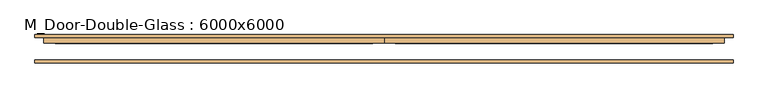
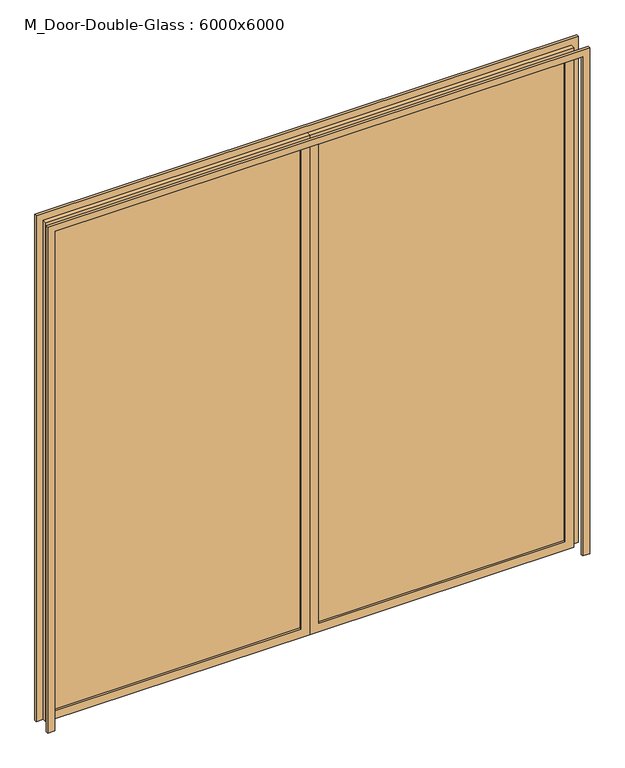
"""IFC4 building model written with IfcOpenShell, lengths in millimetres: door geometry, M_Door-Double-Glass : 6000x6000."""

from ifc_helpers import new_model, si_unit, frame, origin, place, context, project, spatial, polyline, outline, extrude, source, transform, mapped, element, save


def m_door_double_glass_6000x6000_a7e1d600(model_context):
    return source(origin(), model_context, "Body", "SweptSolid", [
        extrude(outline(polyline([(6000.0, -3000.0), (0.0, -3000.0), (0.0, 0.0), (6000.0, 0.0), (6000.0, -3000.0)]), holes=[polyline([(5900.0, -2900.0), (5900.0, -100.0), (100.0, -100.0), (100.0, -2900.0), (5900.0, -2900.0)])]), frame((0.0, 52.38125, 0.0), z_axis=(0.0, 1.0, 0.0), x_axis=(0.0, 0.0, 1.0)), (0.0, 0.0, 1.0), 50.0),
        extrude(outline(polyline([(6000.0, 3000.0), (6000.0, 0.0), (0.0, 0.0), (0.0, 3000.0), (6000.0, 3000.0)]), holes=[polyline([(5900.0, 2900.0), (100.0, 2900.0), (100.0, 100.0), (5900.0, 100.0), (5900.0, 2900.0)])]), frame((0.0, 52.38125, 0.0), z_axis=(0.0, 1.0, 0.0), x_axis=(0.0, 0.0, 1.0)), (0.0, 0.0, 1.0), 50.0),
        extrude(outline(polyline([(100.0, 80.55625), (2900.0, 80.55625), (2900.0, 74.20625), (100.0, 74.20625), (100.0, 80.55625)])), frame((0.0, 0.0, 100.0), z_axis=(0.0, 0.0, 1.0), x_axis=(1.0, 0.0, 0.0)), (0.0, 0.0, 1.0), 5800.0),
        extrude(outline(polyline([(-2900.0, 80.55625), (-100.0, 80.55625), (-100.0, 74.20625), (-2900.0, 74.20625), (-2900.0, 80.55625)])), frame((0.0, 0.0, 100.0), z_axis=(0.0, 0.0, 1.0), x_axis=(1.0, 0.0, 0.0)), (0.0, 0.0, 1.0), 5800.0),
        extrude(outline(polyline([(0.0, 3080.0), (6080.0, 3080.0), (6080.0, -3080.0), (0.0, -3080.0), (0.0, -3000.0), (6000.0, -3000.0), (6000.0, 3000.0), (0.0, 3000.0), (0.0, 3080.0)])), frame((0.0, 102.38125, 0.0), z_axis=(0.0, 1.0, 0.0), x_axis=(0.0, 0.0, 1.0)), (0.0, 0.0, 1.0), 25.0),
        extrude(outline(polyline([(0.0, 3080.0), (6080.0, 3080.0), (6080.0, -3080.0), (0.0, -3080.0), (0.0, -3000.0), (6000.0, -3000.0), (6000.0, 3000.0), (0.0, 3000.0), (0.0, 3080.0)])), frame((0.0, -122.61875, 0.0), z_axis=(0.0, 1.0, 0.0), x_axis=(0.0, 0.0, 1.0)), (0.0, 0.0, 1.0), 25.0),
    ])


if __name__ == "__main__":
    model = new_model("IFC4")
    model_context = context("Model", 3, world=origin())
    ifc_project = project(units=[si_unit("LENGTHUNIT", "METRE", prefix="MILLI")], contexts=[model_context])
    site = spatial("IfcSite", under=ifc_project)
    building = spatial("IfcBuilding", under=site)
    placement = place(None, origin())
    m_door_double_glass_6000x6000_shape = m_door_double_glass_6000x6000_a7e1d600(model_context)
    element("IfcDoor", 1, ObjectType="M_Door-Double-Glass : 6000x6000", at=placement, inside=building, context=model_context, shape_type="MappedRepresentation", body=[
        mapped(m_door_double_glass_6000x6000_shape, transform((0.0, 0.0, 0.0), x_axis=(1.0, 0.0, 0.0), y_axis=(0.0, 1.0, 0.0), z_axis=(0.0, 0.0, 1.0))),
    ])
    save(model, "model.ifc")

# Revit data of these elements
# Type "M_Door-Double-Glass : 6000x6000"
#   Type Mark = "22"
#   Construction Type Id = "opn-d45"
#   Assembly Code = "C1020"
#   Analytic Construction = "Wood frame, double glass door "
#   W = 3000 mm
#   Thickness = 50 mm
#   Thermal Resistance (R) = 0.31964 (m²·K)/W
#   Swing Angle [instance default] = 90.00°
#   Heat Transfer Coefficient (U) = 3.12872 W/(m²·K)
#   Height = 6000 mm
#   Bottom Rail = 100 mm
#   Top Rail = 100 mm
#   Stiles = 100 mm
#   Trim Projection = 25 mm
#   Trim Width = 80 mm
#   Width = 6000 mm
#   Glazing = Glass
#   Panel Material = Wood - Birch - Solid Stained Light Low Gloss
#   Trim Material = Paint - Sienna
#   Visual Light Transmittance = 0
#   Solar Heat Gain Coefficient = 0
#   Function = (empty or 0)
#   Wall Closure = (empty or 0)
# Element 1 (IfcDoor, "M_Door-Double-Glass : 6000x6000")
#   Materials on its faces: "Wood - Birch - Solid Stained Light Low Gloss", "Paint - Sienna", "Glass"
# Materials
#   "Glass": class "Glass", colour RGB 0 128 192, transparency 0.75, Description = "Soda Lime Glass", Cost = 0
#   "Wood - Birch - Solid Stained Light Low Gloss": class "Wood", colour RGB 210 159 95, transparency 0, Cost = 0
#   "Paint - Sienna": class "Miscellaneous", colour RGB 118 70 51, transparency 0, Cost = 0
